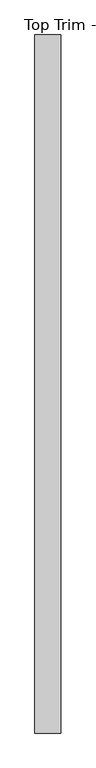
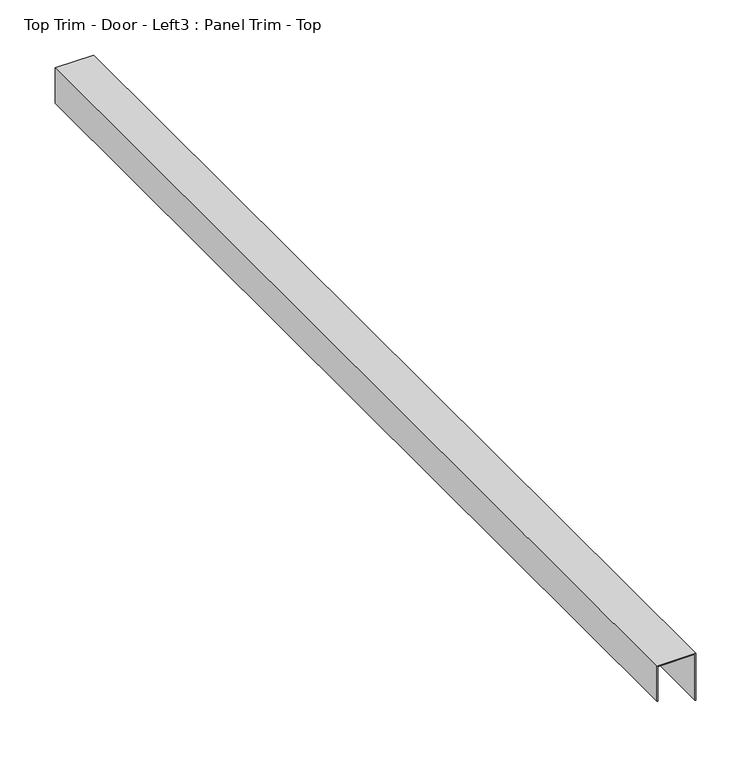
"""IFC4 building model written with IfcOpenShell, lengths in millimetres: proxy geometry, Top Trim - Door - Left3 : Panel Trim - Top."""

from ifc_helpers import new_model, si_unit, frame, origin, place, context, project, spatial, polyline, outline, extrude, source, transform, mapped, element, save


def top_trim_door_left3_panel_trim_top_50f9c082(model_context):
    return source(origin(), model_context, "Body", "SweptSolid", [
        extrude(outline(polyline([(2438.4, 587327.0060739), (2438.4, 587365.8934739), (2387.6, 587365.8934739), (2387.6, 587366.6808739), (2439.19375, 587366.6808739), (2439.19375, 587326.2186739), (2400.3, 587326.2186739), (2400.3, 587327.0060739), (2438.4, 587327.0060739)])), frame((0.0, -535201.5663841, 0.0), z_axis=(0.0, 1.0, 0.0), x_axis=(0.0, 0.0, 1.0)), (0.0, 0.0, 1.0), 1092.2),
    ])


if __name__ == "__main__":
    model = new_model("IFC4")
    model_context = context("Model", 3, world=origin())
    ifc_project = project(units=[si_unit("LENGTHUNIT", "METRE", prefix="MILLI")], contexts=[model_context])
    site = spatial("IfcSite", under=ifc_project)
    building = spatial("IfcBuilding", under=site)
    placement = place(None, origin())
    top_trim_door_left3_panel_trim_top_shape = top_trim_door_left3_panel_trim_top_50f9c082(model_context)
    element("IfcBuildingElementProxy", 1, Name="Top Trim - Door - Left3 : Panel Trim - Top", ObjectType="Top Trim - Door - Left3 : Panel Trim - Top", at=placement, inside=building, context=model_context, shape_type="MappedRepresentation", body=[
        mapped(top_trim_door_left3_panel_trim_top_shape, transform((0.0, 0.0, 0.0), x_axis=(1.0, 0.0, 0.0), y_axis=(0.0, 1.0, 0.0), z_axis=(0.0, 0.0, 1.0))),
    ])
    save(model, "model.ifc")

# Revit data of these elements
# Element 1 (IfcBuildingElementProxy, "Top Trim - Door - Left3 : Panel Trim - Top")
#   Materials on its faces: "EDGE TRIM BY MTL PANEL MFR."
# Materials
#   "EDGE TRIM BY MTL PANEL MFR.": class "Generic", colour RGB 239 242 240, transparency 0, Cost = 0
